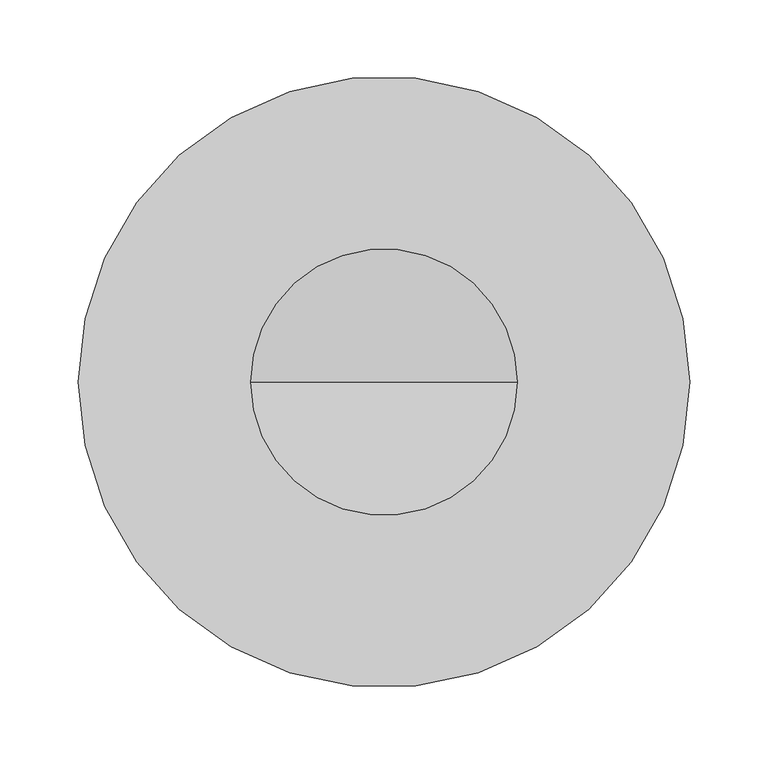
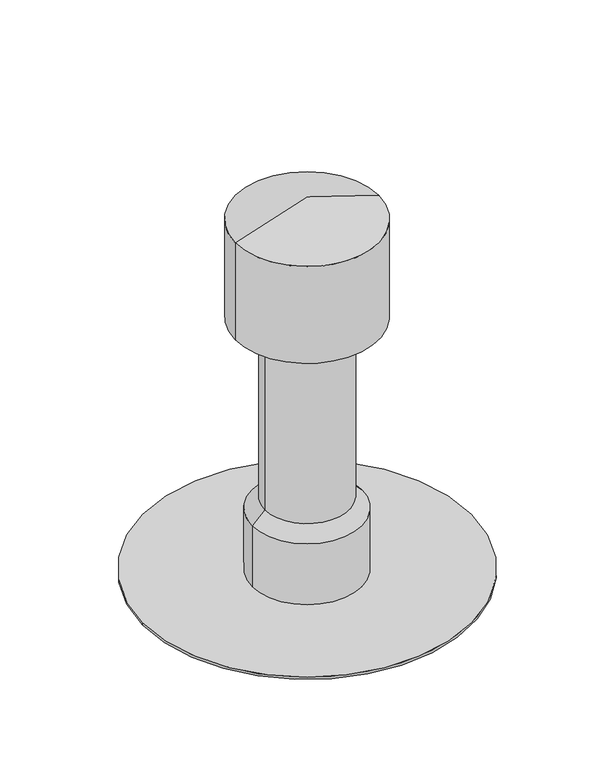
"""IFC4 building model written with IfcOpenShell, lengths in millimetres: proxy geometry, TN_Аэратор кровельный ТехноНИКОЛЬ ЭКО_Тип 2 : Аэратор кровельный ТехноНИКОЛЬ ЭКО 110x470мм."""

from ifc_helpers import new_model, si_unit, point, frame, origin, origin_with_axes, origin_2d, place, context, project, spatial, polyline, circle_curve, trimmed, segment, composite_curve, outline, extrude, source, transform, mapped, element, save
from ifc_brep_helpers import plane_surface, cylinder_surface, revolved_surface, advanced_brep


def specialty_equipment_ef6c45d2(model_context):
    return source(origin(), model_context, "Body", "SolidModel", [
        advanced_brep(
        [(50.0, 0.0, 320.0), (-50.0, 0.0, 320.0), (0.0, 0.0, 320.0), (0.0, 0.0, 3.0), (-65.0, 0.0, 3.0), (65.0, 0.0, 3.0), (50.0, 0.0, 94.4213562), (-50.0, 0.0, 94.4213562), (65.0, 0.0, 79.4213562), (-65.0, 0.0, 79.4213562)],
        [
            (0, 1, circle_curve(frame((0.0, 0.0, 320.0), z_axis=(0.0, 0.0, 1.0), x_axis=(-1.0, 0.0, 0.0)), 50.0)),
            (1, 2),
            (2, 0),
            (1, 0, circle_curve(frame((0.0, 0.0, 320.0), z_axis=(0.0, 0.0, 1.0), x_axis=(-1.0, 0.0, 0.0)), 50.0)),
            (3, 4),
            (4, 5, circle_curve(frame((0.0, 0.0, 3.0), z_axis=(0.0, 0.0, -1.0), x_axis=(-1.0, 0.0, 0.0)), 65.0)),
            (5, 3),
            (5, 4, circle_curve(frame((0.0, 0.0, 3.0), z_axis=(0.0, 0.0, -1.0), x_axis=(-1.0, 0.0, 0.0)), 65.0)),
            (6, 7, circle_curve(frame((0.0, 0.0, 94.4213562), z_axis=(0.0, 0.0, 1.0), x_axis=(-1.0, 0.0, 0.0)), 50.0)),
            (7, 1),
            (0, 6),
            (7, 6, circle_curve(frame((0.0, 0.0, 94.4213562), z_axis=(0.0, 0.0, 1.0), x_axis=(-1.0, 0.0, 0.0)), 50.0)),
            (8, 9, circle_curve(frame((0.0, 0.0, 79.4213562), z_axis=(0.0, 0.0, 1.0), x_axis=(-1.0, 0.0, 0.0)), 65.0)),
            (9, 7),
            (6, 8),
            (9, 8, circle_curve(frame((0.0, 0.0, 79.4213562), z_axis=(0.0, 0.0, 1.0), x_axis=(-1.0, 0.0, 0.0)), 65.0)),
            (4, 9),
            (8, 5),
        ],
        [
            plane_surface(frame((0.0, 0.0, 320.0), z_axis=(0.0, 0.0, 1.0), x_axis=(-1.0, 0.0, 0.0))),
            plane_surface(frame((0.0, 0.0, 3.0), z_axis=(0.0, 0.0, -1.0), x_axis=(-1.0, 0.0, 0.0))),
            cylinder_surface(frame((0.0, 0.0, -2.0), z_axis=(0.0, 0.0, -1.0), x_axis=(-1.0, 0.0, 0.0)), 50.0),
            revolved_surface(polyline([(-50.0, 0.0, 94.4213562), (-65.0, 0.0, 79.4213562)]), (0.0, 0.0, -2.0), (0.0, 0.0, -1.0)),
            cylinder_surface(frame((0.0, 0.0, -2.0), z_axis=(0.0, 0.0, -1.0), x_axis=(-1.0, 0.0, 0.0)), 65.0),
        ],
        [
            (0, [[1, 2, 3]]),
            (0, [[4, -3, -2]]),
            (1, [[5, 6, 7]]),
            (1, [[-7, 8, -5]]),
            (2, [[9, 10, -1, 11]]),
            (2, [[12, -11, -4, -10]]),
            (3, [[13, 14, -9, 15]]),
            (3, [[16, -15, -12, -14]]),
            (4, [[-6, 17, -13, 18]]),
            (4, [[-8, -18, -16, -17]]),
        ],
    ),
        advanced_brep(
        [(0.0, 0.0, 320.0), (-85.0, 0.0, 320.0), (85.0, 0.0, 320.0), (-85.0, 0.0, 441.6666667), (85.0, 0.0, 441.6666667), (0.0, 0.0, 470.0)],
        [
            (0, 1),
            (1, 2, circle_curve(frame((0.0, 0.0, 320.0), z_axis=(0.0, 0.0, -1.0), x_axis=(-1.0, 0.0, 0.0)), 85.0)),
            (2, 0),
            (2, 1, circle_curve(frame((0.0, 0.0, 320.0), z_axis=(0.0, 0.0, -1.0), x_axis=(-1.0, 0.0, 0.0)), 85.0)),
            (1, 3),
            (3, 4, circle_curve(frame((0.0, 0.0, 441.6666667), z_axis=(0.0, 0.0, -1.0), x_axis=(-1.0, 0.0, 0.0)), 85.0)),
            (4, 2),
            (4, 3, circle_curve(frame((0.0, 0.0, 441.6666667), z_axis=(0.0, 0.0, -1.0), x_axis=(-1.0, 0.0, 0.0)), 85.0)),
            (3, 5),
            (5, 4),
        ],
        [
            plane_surface(frame((0.0, 0.0, 320.0), z_axis=(0.0, 0.0, -1.0), x_axis=(-1.0, 0.0, 0.0))),
            cylinder_surface(frame((0.0, 0.0, 485.0), z_axis=(0.0, 0.0, -1.0), x_axis=(-1.0, 0.0, 0.0)), 85.0),
            revolved_surface(polyline([(0.0, 0.0, 470.0), (-85.0, 0.0, 441.6666667)]), (0.0, 0.0, 485.0), (0.0, 0.0, -1.0)),
        ],
        [
            (0, [[1, 2, 3]]),
            (0, [[-3, 4, -1]]),
            (1, [[-2, 5, 6, 7]]),
            (1, [[-4, -7, 8, -5]]),
            (2, [[-6, 9, 10]]),
            (2, [[-8, -10, -9]]),
        ],
    ),
        extrude(outline(composite_curve([segment(trimmed(circle_curve(origin_2d(), 195.0), [point((-195.0, 0.0))], [point((195.0, 0.0))], False, "CARTESIAN"), True, "CONTINUOUS"), segment(trimmed(circle_curve(origin_2d(), 195.0), [point((195.0, 0.0))], [point((-195.0, 0.0))], False, "CARTESIAN"), True, "CONTINUOUS")], self_intersect=False)), origin_with_axes(), (0.0, 0.0, 1.0), 3.0),
    ])


if __name__ == "__main__":
    model = new_model("IFC4")
    model_context = context("Model", 3, world=origin())
    ifc_project = project(units=[si_unit("LENGTHUNIT", "METRE", prefix="MILLI")], contexts=[model_context])
    site = spatial("IfcSite", under=ifc_project)
    building = spatial("IfcBuilding", under=site)
    placement = place(None, origin())
    specialty_equipment_shape = specialty_equipment_ef6c45d2(model_context)
    element("IfcBuildingElementProxy", 1, Name="TN_Аэратор кровельный ТехноНИКОЛЬ ЭКО_Тип 2 : Аэратор кровельный ТехноНИКОЛЬ ЭКО 110x470мм", ObjectType="TN_Аэратор кровельный ТехноНИКОЛЬ ЭКО_Тип 2 : Аэратор кровельный ТехноНИКОЛЬ ЭКО 110x470мм", at=placement, inside=building, context=model_context, shape_type="MappedRepresentation", body=[
        mapped(specialty_equipment_shape, transform((0.0, 0.0, 0.0), x_axis=(1.0, 0.0, 0.0), y_axis=(0.0, 1.0, 0.0), z_axis=(0.0, 0.0, 1.0))),
    ])
    save(model, "model.ifc")

# Revit data of these elements
# Type "TN_Аэратор кровельный ТехноНИКОЛЬ ЭКО_Тип 2 : Аэратор кровельный ТехноНИКОЛЬ ЭКО 110x470мм"
#   Description = "Аэратор предназначен для удаления излишек влаги из кровельного пирога, что позволяет избежать накопления влаги и вздутий под кровельным материалом.\r\nРекомендуется устанавливать 1 аэратор на 100-150 м2 кровельного покрытия."
#   Manufacturer = "ТехноНИКОЛЬ"
#   ADSK_Обозначение = "ТехноНИКОЛЬ"
#   ADSK_Наименование = "Аэратор кровельный ТехноНИКОЛЬ ЭКО 110x470мм"
#   ADSK_Код изделия = "1758"
#   ADSK_Завод-изготовитель = "ТехноНИКОЛЬ"
#   ADSK_Единица измерения = "шт."
#   ADSK_Группирование = "Комплектующие и воронки"
#   ADSK_URL страницы изделия = ""
#   ADSK_URL документации изделия = ""
#   ADSK_Размер_Ширина = 50 mm
#   ADSK_Размер_Высота = 470 mm
#   ADSK_Количество = 1
#   Материал = TN_ПВХ_Черный
#   Default Elevation = 0
#   URL = ""
# Element 1 (IfcBuildingElementProxy, "TN_Аэратор кровельный ТехноНИКОЛЬ ЭКО_Тип 2 : Аэратор кровельный ТехноНИКОЛЬ ЭКО 110x470мм")
#   Materials on its faces: "TN_ПВХ_Черный"
# Materials
#   "TN_ПВХ_Черный": class "Типовые", colour RGB 48 48 48, transparency 0, Cost = 0
